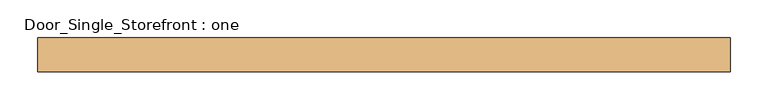
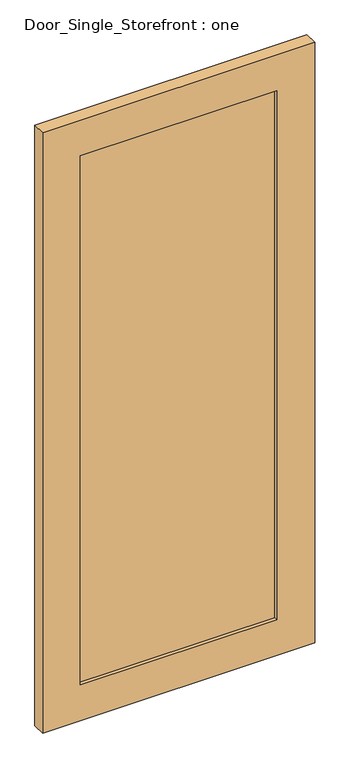
"""IFC4 building model written with IfcOpenShell, lengths in millimetres: door geometry, Door_Single_Storefront : one."""

from ifc_helpers import new_model, si_unit, frame, origin, place, context, project, spatial, polyline, outline, extrude, source, transform, mapped, element, save


def door_single_storefront_one_05824156(model_context):
    return source(origin(), model_context, "Body", "SweptSolid", [
        extrude(outline(polyline([(330.2, 6.35), (330.2, -12.7), (-330.2, -12.7), (-330.2, 6.35), (330.2, 6.35)])), frame((0.0, 0.0, 127.0), z_axis=(0.0, 0.0, 1.0), x_axis=(1.0, 0.0, 0.0)), (0.0, 0.0, 1.0), 1879.6),
        extrude(outline(polyline([(2133.6, -457.2), (0.0, -457.2), (0.0, 457.2), (2133.6, 457.2), (2133.6, -457.2)]), holes=[polyline([(127.0, 330.2), (127.0, -330.2), (2006.6, -330.2), (2006.6, 330.2), (127.0, 330.2)])]), frame((0.0, -25.4, 0.0), z_axis=(0.0, 1.0, 0.0), x_axis=(0.0, 0.0, 1.0)), (0.0, 0.0, 1.0), 44.45),
    ])


if __name__ == "__main__":
    model = new_model("IFC4")
    model_context = context("Model", 3, world=origin())
    ifc_project = project(units=[si_unit("LENGTHUNIT", "METRE", prefix="MILLI")], contexts=[model_context])
    site = spatial("IfcSite", under=ifc_project)
    building = spatial("IfcBuilding", under=site)
    placement = place(None, origin())
    door_single_storefront_one_shape = door_single_storefront_one_05824156(model_context)
    element("IfcDoor", 1, ObjectType="Door_Single_Storefront : one", at=placement, inside=building, context=model_context, shape_type="MappedRepresentation", body=[
        mapped(door_single_storefront_one_shape, transform((0.0, 0.0, 0.0), x_axis=(1.0, 0.0, 0.0), y_axis=(0.0, 1.0, 0.0), z_axis=(0.0, 0.0, 1.0))),
    ])
    save(model, "model.ifc")

# Revit data of these elements
# Type "Door_Single_Storefront : one"
#   Type Mark = "29"
#   Analytic Construction = "<None>"
#   Stile_Width = 0' - 5"
#   Door_Thickness = 0' - 1 3/4"
#   Door_Offset = 0' - 1"
#   Glass_Material = INSULATED GLAZING
#   Frame_Material = ALUMINUM STOREFRONT
#   Function = (empty or 0)
# Element 1 (IfcDoor, "Door_Single_Storefront : one")
#   Materials on its faces: "ALUMINUM STOREFRONT", "INSULATED GLAZING"
# Materials
#   "INSULATED GLAZING": class "Glass", colour RGB 196 205 210, transparency 0.85, Description = "Soda Lime Glass", Cost = 0
#   "ALUMINUM STOREFRONT": class "Metal", colour RGB 244 244 244, transparency 0, Description = "Aluminum 6061", Cost = 0
